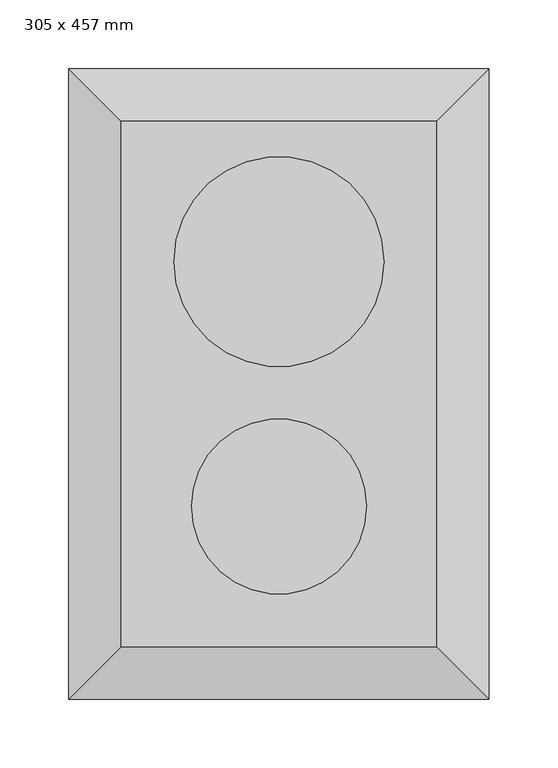
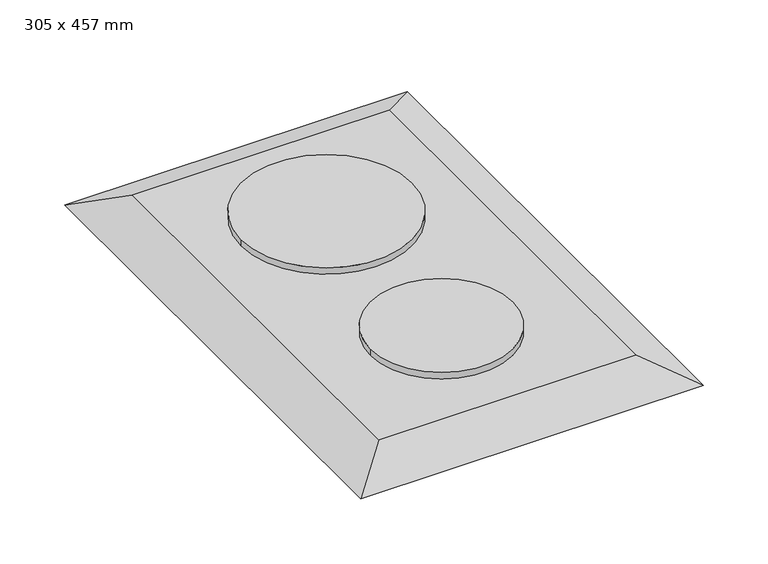
"""IFC4 building model written with IfcOpenShell, lengths in millimetres: proxy geometry, Cocina encimera - 2 fuegos : 305 x 457 mm."""

import ifcopenshell
import ifcopenshell.guid

model = None  # the IFC model being written
_history = None  # IfcOwnerHistory: only IFC2X3 demands one
_inside = {}  # id of a spatial element -> (the spatial element, [elements in it])
_under = {}  # id of a project, library or spatial element -> (it, [spatial elements below it])
_declared = {}  # id of a project -> (the project, [libraries it declares])
_typed = {}  # id of a type object -> (the type object, [elements of that type])
_made_of = {}  # id of a material, layer set ... -> (it, [elements and type objects made of it])


def new_model(schema):
    """Start an empty IFC model of exactly this schema.

    Asked for "IFC4X3", IfcOpenShell would pick the latest addendum, in which some entities
    have other attributes; the version numbers below select the first issue.
    IFC2X3 requires an IfcOwnerHistory on every rooted entity: one is made here for all.
    """
    global model, _history
    if schema == "IFC4X3":
        model = ifcopenshell.file(schema_version=(4, 3, 0, 0))
    else:
        model = ifcopenshell.file(schema=schema)
    _inside.clear()
    _under.clear()
    _declared.clear()
    _typed.clear()
    _made_of.clear()
    _history = None
    if model.schema == "IFC2X3":
        org = make("IfcOrganization", Name="unknown")
        user = make(
            "IfcPersonAndOrganization",
            ThePerson=make("IfcPerson", FamilyName="unknown"),
            TheOrganization=org,
        )
        app = make(
            "IfcApplication",
            ApplicationDeveloper=org,
            Version="unknown",
            ApplicationFullName="unknown",
            ApplicationIdentifier="unknown",
        )
        _history = make(
            "IfcOwnerHistory",
            OwningUser=user,
            OwningApplication=app,
            ChangeAction="ADDED",
            CreationDate=0,
        )
    return model


def make(cls, **values):
    """One entity of the class cls with the attributes given. An attribute that is None is left unset."""
    return model.create_entity(
        cls, **{name: value for name, value in values.items() if value is not None}
    )


def rooted(cls, **values):
    """An entity with a GlobalId (a new one), such as an element, a storey or a relation."""
    return make(cls, GlobalId=ifcopenshell.guid.new(), OwnerHistory=_history, **values)


def si_unit(unit_type, name, prefix=None):
    """IfcSIUnit, for example si_unit("LENGTHUNIT", "METRE", prefix="MILLI")."""
    return make("IfcSIUnit", UnitType=unit_type, Prefix=prefix, Name=name)


def assignment(units):
    """IfcUnitAssignment: the units of a project."""
    return None if units is None else make("IfcUnitAssignment", Units=units)


def point(xyz):
    """IfcCartesianPoint."""
    return None if xyz is None else make("IfcCartesianPoint", Coordinates=xyz)


def direction(xyz):
    """IfcDirection."""
    return None if xyz is None else make("IfcDirection", DirectionRatios=xyz)


def frame(location, z_axis=None, x_axis=None):
    """IfcAxis2Placement3D, a coordinate frame: its origin and axes. An axis left out is left unset."""
    return make(
        "IfcAxis2Placement3D",
        Location=point(location),
        Axis=direction(z_axis),
        RefDirection=direction(x_axis),
    )


def frame_2d(location, x_axis=None):
    """IfcAxis2Placement2D, a coordinate frame in the plane: its origin and x axis."""
    return make(
        "IfcAxis2Placement2D", Location=point(location), RefDirection=direction(x_axis)
    )


def origin():
    """The frame at (0, 0, 0) with its axes left unset."""
    return frame((0.0, 0.0, 0.0))


def place(relative_to, where):
    """IfcLocalPlacement: puts the frame where relative to a parent placement (None: the world)."""
    return make(
        "IfcLocalPlacement", PlacementRelTo=relative_to, RelativePlacement=where
    )


def context(
    kind, dimensions, precision=None, world=None, true_north=None, identifier=None
):
    """IfcGeometricRepresentationContext, for example the 3D "Model" context."""
    return make(
        "IfcGeometricRepresentationContext",
        ContextIdentifier=identifier,
        ContextType=kind,
        CoordinateSpaceDimension=dimensions,
        Precision=precision,
        WorldCoordinateSystem=world,
        TrueNorth=true_north,
    )


def project(units=None, contexts=None):
    """IfcProject with its units and contexts."""
    return rooted(
        "IfcProject",
        Name="project",
        RepresentationContexts=contexts,
        UnitsInContext=assignment(units),
    )


def spatial(cls, under=None, at=None, **own):
    """A site, building, storey or space (cls), placed at a placement, below another one or the project."""
    s = rooted(cls, ObjectPlacement=at, **own)
    if under is not None:
        _under.setdefault(under.id(), (under, []))[1].append(s)
    return s


def circle_curve(where, radius):
    """IfcCircle in the frame where."""
    return make("IfcCircle", Position=where, Radius=radius)


def trimmed(basis, trim1, trim2, sense, master):
    """IfcTrimmedCurve: the piece of a basis curve between two trims."""
    return make(
        "IfcTrimmedCurve",
        BasisCurve=basis,
        Trim1=trim1,
        Trim2=trim2,
        SenseAgreement=sense,
        MasterRepresentation=master,
    )


def segment(curve, same_sense, transition):
    """IfcCompositeCurveSegment."""
    return make(
        "IfcCompositeCurveSegment",
        Transition=transition,
        SameSense=same_sense,
        ParentCurve=curve,
    )


def composite_curve(segments, self_intersect=None):
    """IfcCompositeCurve: segments joined end to end."""
    return make("IfcCompositeCurve", Segments=segments, SelfIntersect=self_intersect)


def outline(outer, holes=None, kind="AREA"):
    """IfcArbitraryClosedProfileDef: a profile drawn as a closed curve; with holes, ...WithVoids."""
    if holes is None:
        return make("IfcArbitraryClosedProfileDef", ProfileType=kind, OuterCurve=outer)
    return make(
        "IfcArbitraryProfileDefWithVoids",
        ProfileType=kind,
        OuterCurve=outer,
        InnerCurves=holes,
    )


def extrude(swept, where, along, depth):
    """IfcExtrudedAreaSolid: the profile swept, set in the frame where, extruded along a direction by depth."""
    return make(
        "IfcExtrudedAreaSolid",
        SweptArea=swept,
        Position=where,
        ExtrudedDirection=direction(along),
        Depth=depth,
    )


def faces_of(points, faces, orient=None, outer=None):
    """IfcFace entities. A face is a list of loops; a loop is a list of indices into points, from 0.

    orient and outer hold one flag for each loop. By default every Orientation is true, the
    first loop of a face is its IfcFaceOuterBound and the others are IfcFaceBound.
    """
    made = []
    for i, loops in enumerate(faces):
        bounds = []
        for j, loop in enumerate(loops):
            is_outer = j == 0 if outer is None else outer[i][j]
            bounds.append(
                make(
                    "IfcFaceOuterBound" if is_outer else "IfcFaceBound",
                    Bound=make("IfcPolyLoop", Polygon=[points[k] for k in loop]),
                    Orientation=True if orient is None else orient[i][j],
                )
            )
        made.append(make("IfcFace", Bounds=bounds))
    return made


def faceted_brep(points, faces, orient=None, outer=None, voids=None):
    """IfcFacetedBrep: a solid bounded by flat faces; with voids (closed shells), ...WithVoids."""
    shared = [point(p) for p in points]
    hull = make("IfcClosedShell", CfsFaces=faces_of(shared, faces, orient, outer))
    if voids is None:
        return make("IfcFacetedBrep", Outer=hull)
    return make(
        "IfcFacetedBrepWithVoids",
        Outer=hull,
        Voids=[
            make(cls, CfsFaces=faces_of(shared, fs, o, b)) for cls, fs, o, b in voids
        ],
    )


def shape(context_of_items, identifier, shape_type, items):
    """IfcShapeRepresentation: the items that make up one representation, for example the "Body"."""
    return make(
        "IfcShapeRepresentation",
        ContextOfItems=context_of_items,
        RepresentationIdentifier=identifier,
        RepresentationType=shape_type,
        Items=items,
    )


def source(mapping_origin, context_of_items, identifier, shape_type, items):
    """IfcRepresentationMap: a shape defined once, which mapped items show again and again."""
    return make(
        "IfcRepresentationMap",
        MappingOrigin=mapping_origin,
        MappedRepresentation=shape(context_of_items, identifier, shape_type, items),
    )


def transform(
    local_origin,
    x_axis=None,
    y_axis=None,
    z_axis=None,
    scale=None,
    scale2=None,
    scale3=None,
    uniform=True,
):
    """IfcCartesianTransformationOperator3D, or its non-uniform kind. x_axis, y_axis, z_axis: its Axis1, 2, 3."""
    if uniform:
        return make(
            "IfcCartesianTransformationOperator3D",
            Axis1=direction(x_axis),
            Axis2=direction(y_axis),
            LocalOrigin=point(local_origin),
            Scale=scale,
            Axis3=direction(z_axis),
        )
    return make(
        "IfcCartesianTransformationOperator3DnonUniform",
        Axis1=direction(x_axis),
        Axis2=direction(y_axis),
        LocalOrigin=point(local_origin),
        Scale=scale,
        Axis3=direction(z_axis),
        Scale2=scale2,
        Scale3=scale3,
    )


def mapped(mapping_source, mapping_target):
    """IfcMappedItem: shows the shape of a source again, moved by a transform."""
    return make(
        "IfcMappedItem", MappingSource=mapping_source, MappingTarget=mapping_target
    )


def made_of(thing, what):
    """Note that an element or type object is made of a material, layer set ...; save() writes the relation."""
    if what is not None:
        _made_of.setdefault(what.id(), (what, []))[1].append(thing)
    return thing


def element(
    cls,
    number,
    at=None,
    inside=None,
    cuts=None,
    type_object=None,
    material=None,
    context=None,
    identifier="Body",
    shape_type=None,
    held_by="IfcProductDefinitionShape",
    body=None,
    shapes=None,
    **own,
):
    """One element of the class cls, such as IfcWall. Its Tag is "e" and its number.

    at: its placement. inside: the storey or other place that contains it. cuts: it is an
    opening in that element (IfcRelVoidsElement). A single representation is given by context,
    identifier, shape_type and body (its items); several are given by shapes. held_by: the class
    of the entity that holds the representations. save() writes the other relations.
    """
    e = rooted(cls, Tag="e%d" % number, ObjectPlacement=at, **own)
    if body is not None:
        shapes = [shape(context, identifier, shape_type, body)]
    if shapes is not None:
        e.Representation = make(held_by, Representations=shapes)
    if inside is not None:
        _inside.setdefault(inside.id(), (inside, []))[1].append(e)
    if cuts is not None:
        rooted(
            "IfcRelVoidsElement", RelatingBuildingElement=cuts, RelatedOpeningElement=e
        )
    if type_object is not None:
        _typed.setdefault(type_object.id(), (type_object, []))[1].append(e)
    return made_of(e, material)


def aggregate(whole, parts):
    """IfcRelAggregates: a whole, such as a stair, and the parts it consists of."""
    return rooted("IfcRelAggregates", RelatingObject=whole, RelatedObjects=parts)


def save(model, path):
    """Write the relations noted so far, then the file.

    IfcRelAggregates (storeys below a building ...), IfcRelContainedInSpatialStructure (elements
    in a storey), IfcRelDefinesByType, IfcRelAssociatesMaterial and IfcRelDeclares: one each for
    every whole, place, type object, material and project.
    """
    for whole, parts in _under.values():
        aggregate(whole, parts)
    for where, things in _inside.values():
        rooted(
            "IfcRelContainedInSpatialStructure",
            RelatedElements=things,
            RelatingStructure=where,
        )
    for kind, things in _typed.values():
        rooted("IfcRelDefinesByType", RelatedObjects=things, RelatingType=kind)
    for what, things in _made_of.values():
        rooted("IfcRelAssociatesMaterial", RelatedObjects=things, RelatingMaterial=what)
    for by, libraries in _declared.values():
        rooted("IfcRelDeclares", RelatingContext=by, RelatedDefinitions=libraries)
    model.write(path)


def proxy_305_x_457_mm_75991893(model_context):
    return source(origin(), model_context, "Body", "SolidModel", [
        faceted_brep([(190.6, 220.6247956, 919.05), (-38.2, 220.6247956, 919.05), (-38.2, -160.1752044, 919.05), (190.6, -160.1752044, 919.05), (228.7, 258.7247956, 900.0), (228.7, -198.2752044, 900.0), (-76.3, -198.2752044, 900.0), (-76.3, 258.7247956, 900.0)], [[[0, 1, 2, 3]], [[4, 5, 6, 7]], [[4, 7, 1, 0]], [[7, 6, 2, 1]], [[6, 5, 3, 2]], [[5, 4, 0, 3]]]),
        extrude(outline(composite_curve([segment(trimmed(circle_curve(frame_2d((76.2, 119.0247956)), 76.2), [point((152.4, 119.0247956))], [point((0.0, 119.0247956))], False, "CARTESIAN"), True, "CONTINUOUS"), segment(trimmed(circle_curve(frame_2d((76.2, 119.0247956)), 76.2), [point((0.0, 119.0247956))], [point((152.4, 119.0247956))], False, "CARTESIAN"), True, "CONTINUOUS")], self_intersect=False)), frame((0.0, 0.0, 919.05), z_axis=(0.0, 0.0, 1.0), x_axis=(1.0, 0.0, 0.0)), (0.0, 0.0, 1.0), 6.35),
        extrude(outline(composite_curve([segment(trimmed(circle_curve(frame_2d((76.2, -58.5752044)), 63.5), [point((139.7, -58.5752044))], [point((12.7, -58.5752044))], False, "CARTESIAN"), True, "CONTINUOUS"), segment(trimmed(circle_curve(frame_2d((76.2, -58.5752044)), 63.5), [point((12.7, -58.5752044))], [point((139.7, -58.5752044))], False, "CARTESIAN"), True, "CONTINUOUS")], self_intersect=False)), frame((0.0, 0.0, 919.05), z_axis=(0.0, 0.0, 1.0), x_axis=(1.0, 0.0, 0.0)), (0.0, 0.0, 1.0), 6.35),
    ])


if __name__ == "__main__":
    model = new_model("IFC4")
    model_context = context("Model", 3, world=origin())
    ifc_project = project(units=[si_unit("LENGTHUNIT", "METRE", prefix="MILLI")], contexts=[model_context])
    site = spatial("IfcSite", under=ifc_project)
    building = spatial("IfcBuilding", under=site)
    placement = place(None, origin())
    proxy_305_x_457_mm_shape = proxy_305_x_457_mm_75991893(model_context)
    element("IfcBuildingElementProxy", 1, Name="Cocina encimera - 2 fuegos : 305 x 457 mm", ObjectType="Cocina encimera - 2 fuegos : 305 x 457 mm", at=placement, inside=building, context=model_context, shape_type="MappedRepresentation", body=[
        mapped(proxy_305_x_457_mm_shape, transform((0.0, 0.0, 0.0), x_axis=(1.0, 0.0, 0.0), y_axis=(0.0, 1.0, 0.0), z_axis=(0.0, 0.0, 1.0))),
    ])
    save(model, "model.ifc")

# Revit data of these elements
# Type "Cocina encimera - 2 fuegos : 305 x 457 mm"
#   Altura de encimera = 0.90 m
#   Profundidad = 0.457 m
#   Anchura = 0.305 m
#   Máscara [instance default] = yes
#   Quemador = Metal - Cromo
#   Cocina encimera = Metal - Acero, Pulido
#   Default Elevation = 0
# Element 1 (IfcBuildingElementProxy, "Cocina encimera - 2 fuegos : 305 x 457 mm")
#   Materials on its faces: "Metal - Acero, Pulido", "Metal - Cromo"
# Materials
#   "Metal - Cromo": class "Metal", colour RGB 17 17 17, transparency 0
#   "Metal - Acero, Pulido": class "Metal", colour RGB 57 57 57, transparency 0
